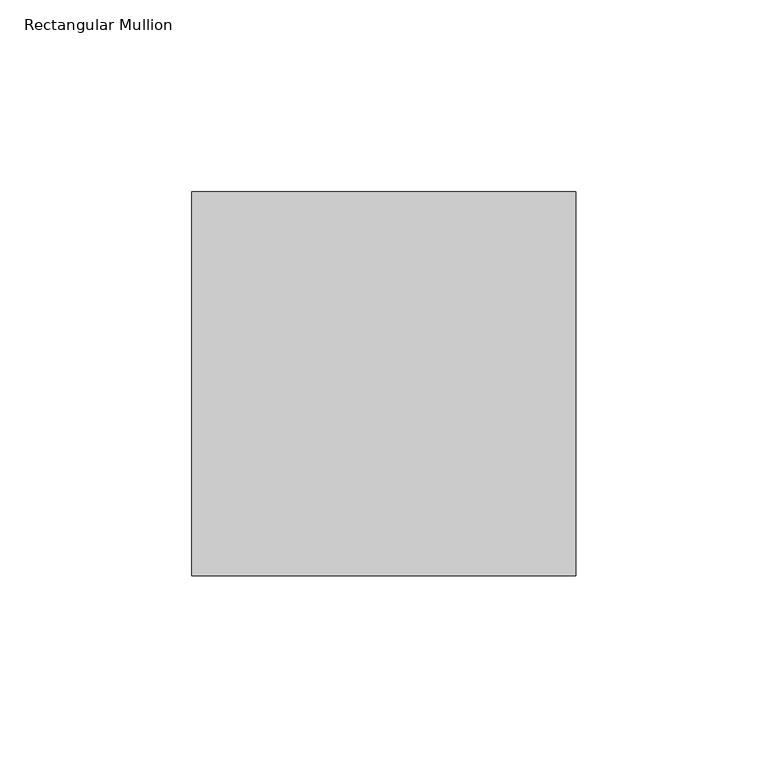
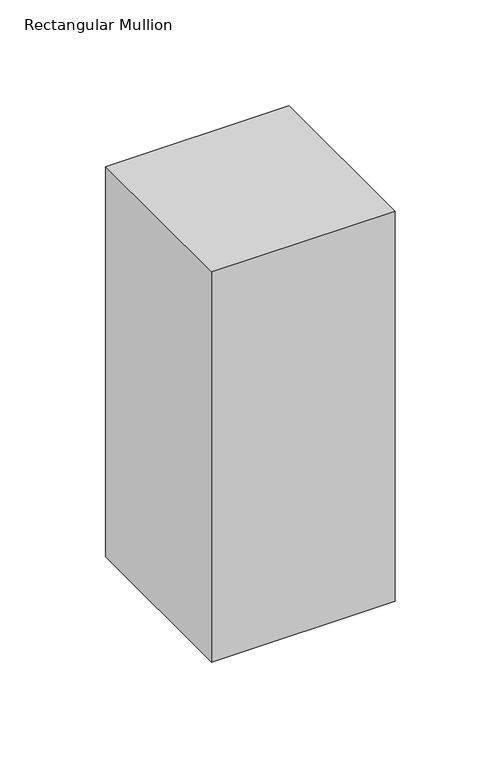
"""IFC4 building model written with IfcOpenShell, lengths in millimetres: member geometry, Rectangular Mullion : 알루미늄_Rectangular Cap_100 x100."""

from ifc_helpers import new_model, si_unit, frame, origin, place, context, project, spatial, polyline, outline, extrude, source, transform, mapped, element, save


def rectangular_mullion_8e76835c(model_context):
    return source(origin(), model_context, "Body", "SweptSolid", [
        extrude(outline(polyline([(0.0, 50.0), (0.0, -50.0), (-100.0, -50.0), (-100.0, 50.0), (0.0, 50.0)])), frame((0.0, 0.0, -225.0000001), z_axis=(0.0, 0.0, 1.0), x_axis=(1.0, 0.0, 0.0)), (0.0, 0.0, 1.0), 225.0000001),
    ])


if __name__ == "__main__":
    model = new_model("IFC4")
    model_context = context("Model", 3, world=origin())
    ifc_project = project(units=[si_unit("LENGTHUNIT", "METRE", prefix="MILLI")], contexts=[model_context])
    site = spatial("IfcSite", under=ifc_project)
    building = spatial("IfcBuilding", under=site)
    placement = place(None, origin())
    rectangular_mullion_shape = rectangular_mullion_8e76835c(model_context)
    element("IfcMember", 1, ObjectType="Rectangular Mullion : 알루미늄_Rectangular Cap_100 x100", at=placement, inside=building, context=model_context, shape_type="MappedRepresentation", body=[
        mapped(rectangular_mullion_shape, transform((0.0, 0.0, 0.0), x_axis=(1.0, 0.0, 0.0), y_axis=(0.0, 1.0, 0.0), z_axis=(0.0, 0.0, 1.0))),
    ])
    save(model, "model.ifc")

# Revit data of these elements
# Type "Rectangular Mullion : 알루미늄_Rectangular Cap_100 x100"
#   built-in parameter 1007304 = 0.328084 (stored number, unit not read)
#   built-in parameter 1007301 = 0.164042 (stored number, unit not read)
#   built-in parameter 1007300 = 0.164042 (stored number, unit not read)
# Element 1 (IfcMember, "Rectangular Mullion : 알루미늄_Rectangular Cap_100 x100")
#   Materials on its faces: "00_Metal_Stainless Steel"
# Materials
#   "00_Metal_Stainless Steel": class "Metal", colour RGB 148 148 148, transparency 0, Description = "Steel", Cost = 0
